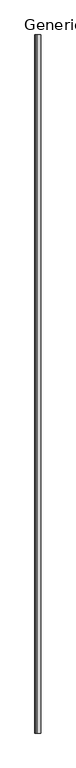
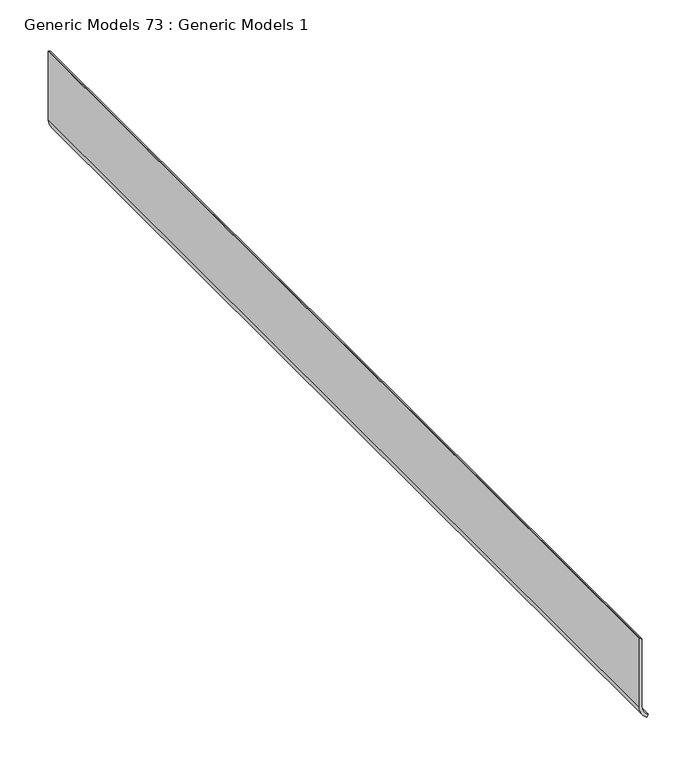
"""IFC4 building model written with IfcOpenShell, lengths in millimetres: proxy geometry, Generic Models 73 : Generic Models 1."""

from ifc_helpers import new_model, si_unit, point, frame, frame_2d, origin, place, context, project, spatial, polyline, circle_curve, trimmed, segment, composite_curve, outline, extrude, source, transform, mapped, element, save


def generic_models_73_generic_models_1_7c4ccb31(model_context):
    return source(origin(), model_context, "Body", "SweptSolid", [
        extrude(outline(composite_curve([segment(polyline([(101.6, 51108.5310187), (15.4496307, 51108.5310187)]), True, "CONTINUOUS"), segment(trimmed(circle_curve(frame_2d((15.4496307, 51126.3707155)), 17.8396968), [point((15.4496307, 51108.5310187))], [point((0.0, 51117.4508671))], False, "CARTESIAN"), True, "CONTINUOUS"), segment(polyline([(0.0, 51117.4508671), (2.7496307, 51119.0383671)]), True, "CONTINUOUS"), segment(trimmed(circle_curve(frame_2d((15.4496307, 51126.3707155)), 14.6646968), [point((2.7496307, 51119.0383671))], [point((15.4496307, 51111.7060187))], True, "CARTESIAN"), True, "CONTINUOUS"), segment(polyline([(15.4496307, 51111.7060187), (99.5131982, 51111.7060187)]), True, "CONTINUOUS"), segment(trimmed(circle_curve(frame_2d((99.5131982, 51109.6192169)), 2.0868018), [point((99.5131982, 51111.7060187))], [point((101.6, 51109.6192169))], False, "CARTESIAN"), True, "CONTINUOUS"), segment(polyline([(101.6, 51109.6192169), (101.6, 51108.5310187)]), True, "CONTINUOUS")], self_intersect=False)), frame((0.0, 0.0, 0.0), z_axis=(0.0, 1.0, 0.0), x_axis=(0.0, 0.0, 1.0)), (0.0, 0.0, 1.0), 1219.2),
    ])


if __name__ == "__main__":
    model = new_model("IFC4")
    model_context = context("Model", 3, world=origin())
    ifc_project = project(units=[si_unit("LENGTHUNIT", "METRE", prefix="MILLI")], contexts=[model_context])
    site = spatial("IfcSite", under=ifc_project)
    building = spatial("IfcBuilding", under=site)
    placement = place(None, origin())
    generic_models_73_generic_models_1_shape = generic_models_73_generic_models_1_7c4ccb31(model_context)
    element("IfcBuildingElementProxy", 1, Name="Generic Models 73 : Generic Models 1", ObjectType="Generic Models 73 : Generic Models 1", at=placement, inside=building, context=model_context, shape_type="MappedRepresentation", body=[
        mapped(generic_models_73_generic_models_1_shape, transform((0.0, 0.0, 0.0), x_axis=(1.0, 0.0, 0.0), y_axis=(0.0, 1.0, 0.0), z_axis=(0.0, 0.0, 1.0))),
    ])
    save(model, "model.ifc")

# Revit data of these elements
# Element 1 (IfcBuildingElementProxy, "Generic Models 73 : Generic Models 1")
#   Materials on its faces: "BASE AS SCHEDULED"
# Materials
#   "BASE AS SCHEDULED": class "Generic", colour RGB 120 120 120, transparency 0, Cost = 0
